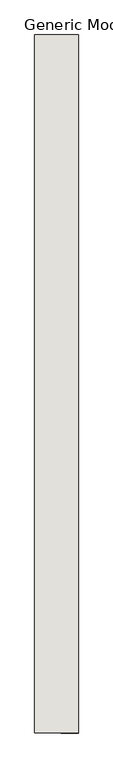
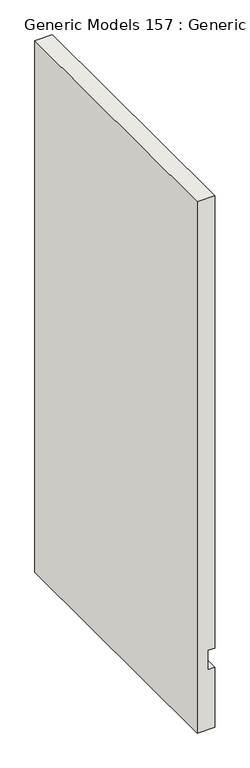
"""IFC4 building model written with IfcOpenShell, lengths in millimetres: wall geometry, Generic Models 157 : Generic Models 1."""

from ifc_helpers import new_model, si_unit, frame, origin, place, context, project, spatial, polyline, outline, extrude, source, transform, mapped, element, save


def generic_models_157_generic_models_1_80720c77(model_context):
    return source(origin(), model_context, "Body", "SweptSolid", [
        extrude(outline(polyline([(16.66875, 141139.8625), (16.66875, 141216.0625), (291.1195631, 141216.0625), (291.1195631, 141185.9), (380.0195631, 141185.9), (380.0195631, 141216.0625), (2455.06875, 141216.0625), (2455.06875, 141139.8625), (16.66875, 141139.8625)])), frame((0.0, 0.0, 0.0), z_axis=(0.0, 1.0, 0.0), x_axis=(0.0, 0.0, 1.0)), (0.0, 0.0, 1.0), 1219.2),
    ])


if __name__ == "__main__":
    model = new_model("IFC4")
    model_context = context("Model", 3, world=origin())
    ifc_project = project(units=[si_unit("LENGTHUNIT", "METRE", prefix="MILLI")], contexts=[model_context])
    site = spatial("IfcSite", under=ifc_project)
    building = spatial("IfcBuilding", under=site)
    placement = place(None, origin())
    generic_models_157_generic_models_1_shape = generic_models_157_generic_models_1_80720c77(model_context)
    element("IfcWall", 1, ObjectType="Generic Models 157 : Generic Models 1", at=placement, inside=building, context=model_context, shape_type="MappedRepresentation", body=[
        mapped(generic_models_157_generic_models_1_shape, transform((0.0, 0.0, 0.0), x_axis=(1.0, 0.0, 0.0), y_axis=(0.0, 1.0, 0.0), z_axis=(0.0, 0.0, 1.0))),
    ])
    save(model, "model.ifc")

# Revit data of these elements
# Element 1 (IfcWall, "Generic Models 157 : Generic Models 1")
#   Materials on its faces: "(S) SOUND BATT. INSULATION (THICKNESS TO MATCH WALL DEPTH)"
# Materials
#   "(S) SOUND BATT. INSULATION (THICKNESS TO MATCH WALL DEPTH)": class "Unassigned", colour RGB 255 255 255, transparency 0, Cost = 0
